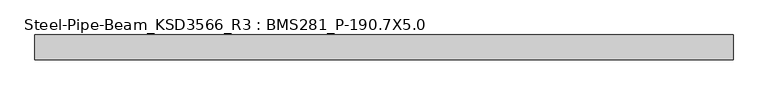
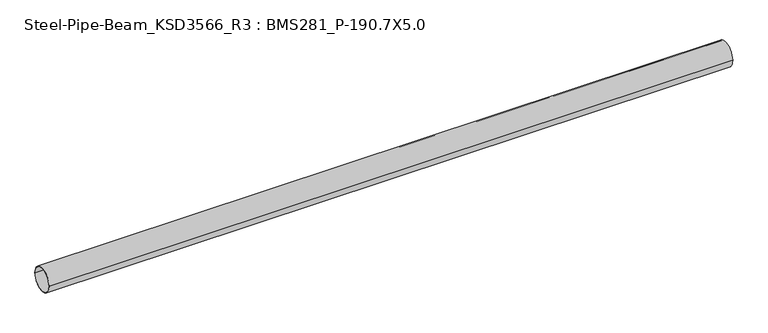
"""IFC4 building model written with IfcOpenShell, lengths in millimetres: member geometry, Steel-Pipe-Beam_KSD3566_R3 : BMS281_P-190.7X5.0."""

from ifc_helpers import new_model, si_unit, point, frame, origin, origin_2d, place, context, project, spatial, circle_curve, trimmed, segment, composite_curve, outline, extrude, source, transform, mapped, element, save


def steel_pipe_beam_ksd3566_r3_bms281_p_190_7x5_0_f0c35028(model_context):
    return source(origin(), model_context, "Body", "SweptSolid", [
        extrude(outline(composite_curve([segment(trimmed(circle_curve(origin_2d(), 95.35), [point((-95.35, 0.0))], [point((95.35, 0.0))], False, "CARTESIAN"), True, "CONTINUOUS"), segment(trimmed(circle_curve(origin_2d(), 95.35), [point((95.35, 0.0))], [point((-95.35, 0.0))], False, "CARTESIAN"), True, "CONTINUOUS")], self_intersect=False), holes=[composite_curve([segment(trimmed(circle_curve(origin_2d(), 90.35), [point((90.35, 0.0))], [point((-90.35, 0.0))], True, "CARTESIAN"), True, "CONTINUOUS"), segment(trimmed(circle_curve(origin_2d(), 90.35), [point((-90.35, 0.0))], [point((90.35, 0.0))], True, "CARTESIAN"), True, "CONTINUOUS")], self_intersect=False)]), frame((-2752.4445734, 0.0, 0.0), z_axis=(1.0, 0.0, 0.0), x_axis=(0.0, 1.0, 0.0)), (0.0, 0.0, 1.0), 5329.8345025),
    ])


if __name__ == "__main__":
    model = new_model("IFC4")
    model_context = context("Model", 3, world=origin())
    ifc_project = project(units=[si_unit("LENGTHUNIT", "METRE", prefix="MILLI")], contexts=[model_context])
    site = spatial("IfcSite", under=ifc_project)
    building = spatial("IfcBuilding", under=site)
    placement = place(None, origin())
    steel_pipe_beam_ksd3566_r3_bms281_p_190_7x5_0_shape = steel_pipe_beam_ksd3566_r3_bms281_p_190_7x5_0_f0c35028(model_context)
    element("IfcMember", 1, ObjectType="Steel-Pipe-Beam_KSD3566_R3 : BMS281_P-190.7X5.0", at=placement, inside=building, context=model_context, shape_type="MappedRepresentation", body=[
        mapped(steel_pipe_beam_ksd3566_r3_bms281_p_190_7x5_0_shape, transform((0.0, 0.0, 0.0), x_axis=(1.0, 0.0, 0.0), y_axis=(0.0, 1.0, 0.0), z_axis=(0.0, 0.0, 1.0))),
    ])
    save(model, "model.ifc")

# Revit data of these elements
# Type "Steel-Pipe-Beam_KSD3566_R3 : BMS281_P-190.7X5.0"
#   Keynote = "P-190.7X5.0"
#   SteelWeight = "Light"
#   t = 0.0050 m
#   Surface Area = 0.599102 m²/m
#   Section Area = 29.1697 cm²
#   Mass per Unit Length = 22.8982 kg/m
#   Length [instance default] = 1.5000 m
#   D = 0.1907 m
#   hec_material4 [instance default] = none
#   hec_material3 [instance default] = none
#   hec_material2 [instance default] = none
#   hec_material1 [instance default] = none
#   Structural Material [instance default] = Steel, 45-345
#   Assembly Code = ""
# Element 1 (IfcMember, "Steel-Pipe-Beam_KSD3566_R3 : BMS281_P-190.7X5.0")
#   Structural Material = none
# Materials
#   "Steel, 45-345": class "Metal", colour RGB 189 187 185, transparency 0, Description = "Steel 345 MPa", Cost = 0
